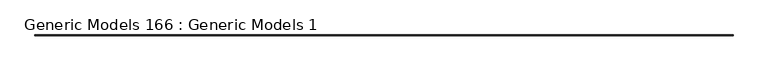
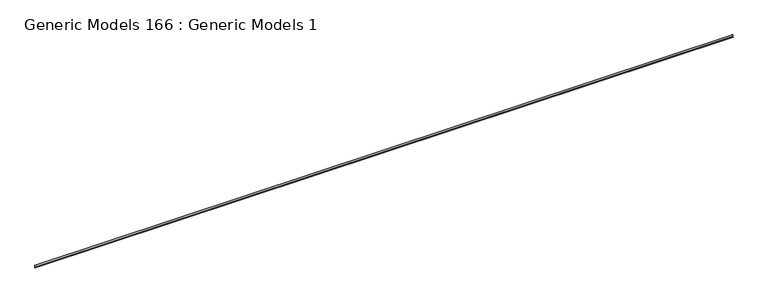
"""IFC4 building model written with IfcOpenShell, lengths in millimetres: proxy geometry, Generic Models 166 : Generic Models 1."""

from ifc_helpers import new_model, si_unit, frame, origin, place, context, project, spatial, polyline, outline, extrude, source, transform, mapped, element, save


def generic_models_166_generic_models_1_f1e5cc8c(model_context):
    return source(origin(), model_context, "Body", "SweptSolid", [
        extrude(outline(polyline([(-28560.7979058, 126996.7728942), (-28539.8429058, 127003.50843), (-28539.8429058, 127047.5728942), (-28538.5729058, 127047.5728942), (-28538.5729058, 127002.5826506), (-28556.6477035, 126996.7728942), (-28539.5361009, 126991.2727363), (-28538.5729058, 126986.1579859), (-28539.8209684, 126985.9229543), (-28540.6442893, 126990.2949461), (-28560.7979058, 126996.7728942)])), frame((-20998.9733045, 0.0, 0.0), z_axis=(1.0, 0.0, 0.0), x_axis=(0.0, 1.0, 0.0)), (0.0, 0.0, 1.0), 19050.0),
    ])


if __name__ == "__main__":
    model = new_model("IFC4")
    model_context = context("Model", 3, world=origin())
    ifc_project = project(units=[si_unit("LENGTHUNIT", "METRE", prefix="MILLI")], contexts=[model_context])
    site = spatial("IfcSite", under=ifc_project)
    building = spatial("IfcBuilding", under=site)
    placement = place(None, origin())
    generic_models_166_generic_models_1_shape = generic_models_166_generic_models_1_f1e5cc8c(model_context)
    element("IfcBuildingElementProxy", 1, Name="Generic Models 166 : Generic Models 1", ObjectType="Generic Models 166 : Generic Models 1", at=placement, inside=building, context=model_context, shape_type="MappedRepresentation", body=[
        mapped(generic_models_166_generic_models_1_shape, transform((0.0, 0.0, 0.0), x_axis=(1.0, 0.0, 0.0), y_axis=(0.0, 1.0, 0.0), z_axis=(0.0, 0.0, 1.0))),
    ])
    save(model, "model.ifc")

# Revit data of these elements
# Element 1 (IfcBuildingElementProxy, "Generic Models 166 : Generic Models 1")
#   Materials on its faces: "_16 GA. COPPER WEEP SCREED W/ MIN. 3 1/2\" ATTACHEMENT FLANGE - LAP UNDERLAYMENT OVER WEED SCREED"
# Materials
#   "_16 GA. COPPER WEEP SCREED W/ MIN. 3 1/2\" ATTACHEMENT FLANGE - LAP UNDERLAYMENT OVER WEED SCREED": class "Generic", colour RGB 253 192 103, transparency 0, Cost = 0
